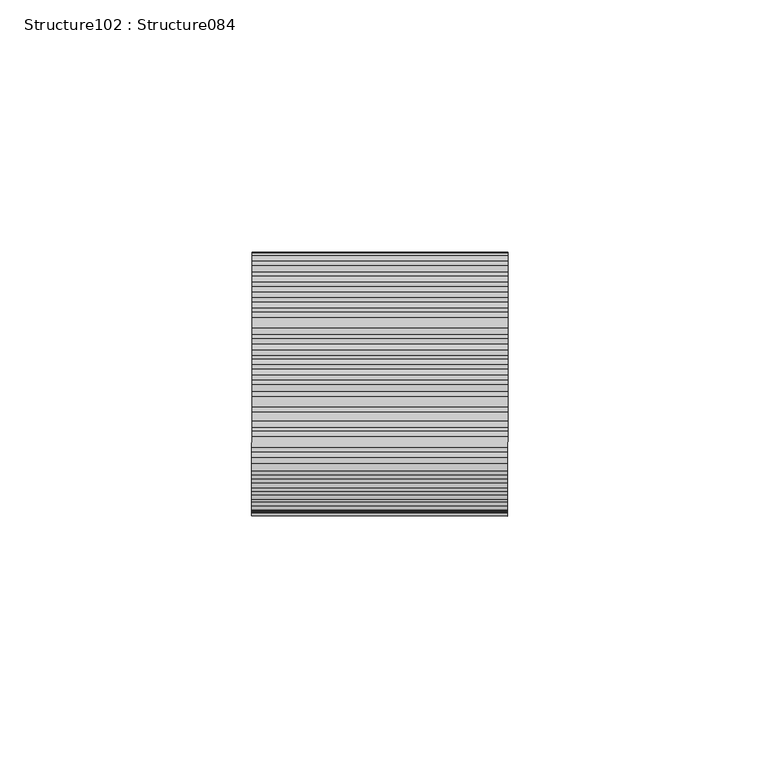
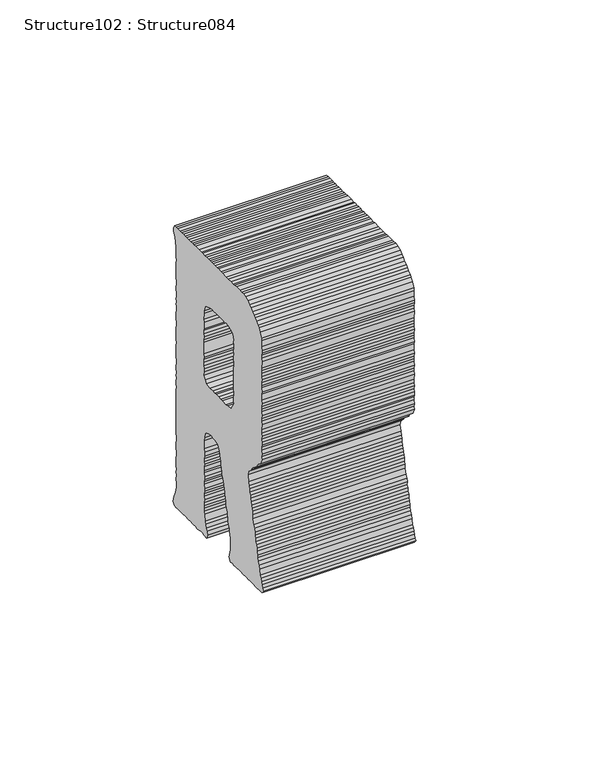
"""IFC4 building model written with IfcOpenShell, lengths in millimetres: proxy geometry, Structure102 : Structure084."""

from ifc_helpers import new_model, si_unit, frame, origin, place, context, project, spatial, polyline, outline, extrude, source, transform, mapped, element, save


def structure102_structure084_8d5e6da8(model_context):
    return source(origin(), model_context, "Body", "SweptSolid", [
        extrude(outline(polyline([(0.7877723, 0.0), (1.9464015, -0.1991228), (2.8602744, -0.2258489), (4.1191818, -0.5725383), (5.014805, -0.7264607), (5.8881786, -1.0119464), (7.2131992, -0.9739456), (7.9618749, -1.2329461), (10.1385127, -1.6070246), (11.3090794, -1.6778663), (12.311293, -1.9804401), (13.2111243, -2.1350857), (14.2117928, -2.4424483), (15.4109212, -2.3828116), (16.5195828, -2.8390667), (17.4342995, -2.8608834), (18.6150357, -2.9334729), (20.3591199, -3.4989322), (21.6394332, -3.7189677), (22.5801144, -3.614914), (23.6845679, -4.0704459), (24.6308599, -3.9673565), (25.7800208, -4.1648521), (26.5039924, -4.5549941), (27.5279624, -4.7309743), (28.8526323, -4.6929132), (29.8357525, -5.1275927), (30.776083, -5.0234788), (32.5416935, -6.2493551), (32.9031424, -7.2342724), (33.5574941, -8.0085019), (34.477038, -8.8236139), (35.0861234, -9.8507291), (35.972525, -11.5876373), (36.8685591, -12.5290416), (37.5229108, -13.303271), (37.9287766, -14.029741), (39.5076035, -14.8278253), (41.6445255, -14.6683322), (42.9644943, -14.6345176), (43.9051754, -14.5304639), (45.0599472, -14.7289238), (46.0220341, -14.4982164), (46.9627152, -14.3941627), (48.1392433, -14.466029), (49.0957798, -14.2340066), (50.041228, -14.1358267), (51.0844997, -14.1847915), (52.1563332, -14.1032778), (53.4327891, -14.3226503), (55.3194114, -14.115447), (56.4288566, -13.7793711), (57.6236345, -13.7240411), (58.7537019, -14.0536423), (59.5858309, -13.7955457), (60.7623592, -13.867412), (61.6189076, -13.4882341), (62.7924221, -13.554528), (63.7358265, -13.4556358), (64.9285003, -13.3999443), (65.8244741, -13.5539269), (66.898061, -13.4727146), (68.1350915, -13.1589264), (69.328609, -13.0983255), (71.318233, -13.0438502), (72.1765349, -12.6649735), (73.2419139, -12.587405), (74.0793029, -12.3302124), (75.2758945, -12.2748331), (76.003044, -11.8734166), (76.8931166, -12.8137963), (76.8480367, -13.8638733), (76.5842472, -14.611004), (76.5400111, -15.6561716), (76.3416115, -16.8105927), (76.0343092, -17.8109105), (75.7045271, -19.7298023), (75.8093424, -20.6702533), (75.3295446, -21.9117003), (75.2811607, -23.7435663), (74.9337097, -25.0027039), (74.4272845, -27.9494233), (74.4005969, -28.8672741), (73.987756, -29.7191213), (74.0707545, -30.7865166), (72.6138584, -31.5939579), (71.7839977, -31.0552851), (70.7821347, -30.7527716), (69.6713689, -30.2961549), (68.9473974, -29.9060129), (66.901912, -29.5544744), (65.7471403, -29.3560146), (64.7624531, -29.7182251), (63.8447229, -29.690836), (62.6738055, -29.6199339), (61.6840006, -29.9762104), (60.4904228, -30.0371621), (59.445047, -29.9878357), (58.3961644, -29.9379066), (57.3516982, -29.893791), (56.362244, -30.2501278), (55.1913266, -30.1792258), (54.145107, -30.1348089), (53.0523006, -30.3383574), (52.1175809, -30.4434355), (51.2156457, -30.2884283), (50.0229718, -30.3441199), (48.9553464, -30.4263568), (47.8617565, -30.634464), (47.0534221, -30.7562085), (45.832477, -30.9427894), (44.914396, -30.91534), (43.7173718, -30.9753383), (42.7766906, -31.079392), (41.494624, -30.8590551), (40.6854459, -30.985709), (39.5926997, -31.1889067), (38.2679695, -31.2273185), (36.4472301, -31.8368423), (35.5455414, -33.266448), (35.3262291, -34.5425532), (34.9408158, -35.2684206), (34.9738469, -36.5929481), (35.1774557, -38.4731762), (35.8364483, -39.2435097), (37.3094464, -39.8927126), (38.4142507, -40.3483048), (41.3574633, -40.8541273), (42.4292967, -40.7726136), (43.70961, -40.9926491), (44.6888727, -41.4266656), (45.7377553, -41.4765946), (46.525177, -41.4765343), (47.5244428, -41.7836559), (48.8103669, -42.0046557), (49.6810775, -42.2846293), (50.8784525, -42.2246912), (51.9076827, -42.4015754), (52.649904, -42.6645211), (53.6552737, -42.9676373), (54.9802942, -42.9296365), (56.0035629, -43.1054961), (56.8555307, -43.5176357), (57.7515045, -43.6716183), (58.9488796, -43.6116803), (60.0554372, -44.0675738), (61.0990598, -44.1165988), (61.869492, -44.2490058), (63.0007539, -44.5737579), (63.9372269, -44.468981), (66.2885299, -44.6124123), (67.125919, -44.3552198), (68.4493124, -44.3266871), (69.3028472, -43.9419367), (70.5019756, -43.8823001), (71.6935756, -44.6185287), (71.3461245, -45.8776663), (70.9132807, -46.8564085), (70.759298, -47.7523823), (70.7307966, -48.6702824), (70.6639602, -49.846953), (70.3566579, -50.8472708), (70.3341179, -51.7661956), (70.157535, -52.7936724), (69.7472914, -53.6409116), (69.69625, -54.689964), (69.3228948, -56.8623937), (69.2778149, -57.9124707), (68.992269, -58.786195), (68.6181303, -60.9631834), (68.5955903, -61.882108), (68.4416077, -62.7780818), (67.1345464, -63.4762478), (66.0458878, -62.8930979), (65.1969939, -62.4861801), (64.1318451, -61.7767379), (63.4057694, -61.3862343), (61.4454907, -60.5179), (60.4218712, -60.34198), (58.3267691, -60.2476341), (57.4807627, -59.8365191), (56.1757452, -59.747625), (55.2985141, -59.4614764), (54.2305381, -59.5436531), (51.2834681, -59.0371676), (50.3063094, -58.6035127), (49.28269, -58.4275928), (47.9738151, -58.3380358), (46.0598327, -58.0090974), (45.0553067, -57.7010718), (44.0334407, -57.5254533), (42.9872211, -57.4810363), (39.0186357, -56.7989926), (37.9732599, -56.7496662), (36.9678902, -56.4465501), (35.6637165, -56.3527465), (34.6422011, -56.1771882), (33.8931746, -55.9181273), (32.8499028, -55.8691626), (31.563628, -55.6481025), (30.5617652, -55.345589), (29.6714021, -55.1925706), (28.7480611, -55.1642173), (27.5989002, -54.9667217), (26.7434256, -54.5539795), (25.5695604, -54.4876253), (24.5262885, -54.4386606), (23.4214843, -53.9830685), (22.6245944, -53.9815015), (21.6235752, -53.6740786), (20.3206618, -53.5855461), (19.2756365, -53.53628), (18.5509637, -53.1460175), (17.268897, -52.9256806), (16.4593683, -53.0522742), (15.300739, -52.8531514), (14.4321325, -52.5735394), (13.3871074, -52.5242734), (12.1225891, -52.1766197), (11.3803678, -51.913674), (10.2086067, -51.8476814), (8.0263581, -51.4726387), (7.2362735, -51.4671869), (6.1085182, -51.1430374), (5.2354954, -50.8576121), (4.0800223, -50.6590317), (3.1400425, -50.7632058), (2.0122874, -50.4390564), (1.0892969, -50.4107633), (-0.1431529, -49.9332339), (-1.1706297, -49.7566511), (-2.2147453, -49.7125957), (-2.9573172, -49.4495897), (-4.0087969, -49.4042688), (-5.0080628, -49.0971472), (-6.2887267, -48.8770514), (-7.1035156, -49.002741), (-8.3620724, -48.6561119), (-9.1102552, -48.3921416), (-10.1314198, -48.2166436), (-11.1997466, -48.29876), (-12.2051163, -47.9956438), (-13.4854295, -47.7756083), (-14.2776182, -47.7697949), (-16.3227529, -47.4183166), (-17.4331681, -46.9617602), (-18.4993908, -47.0442382), (-19.6267952, -46.720149), (-20.6781325, -46.6697981), (-21.5523499, -46.3892219), (-23.7729936, -46.2733003), (-24.8401259, -46.3505675), (-25.6975181, -46.7346549), (-26.7864672, -46.9388664), (-27.9612419, -46.8673015), (-28.903386, -46.1836923), (-28.8523447, -45.1346398), (-28.6983018, -44.2383154), (-28.3526042, -42.9788764), (-28.220378, -42.2094962), (-28.1483637, -41.0384089), (-27.8679957, -40.1591013), (-27.8177379, -39.1146076), (-27.6201821, -37.965096), (-27.3406578, -37.0906979), (-27.2677998, -35.9147012), (-27.010032, -35.1668965), (-26.9597742, -34.1224028), (-26.6073919, -32.0720079), (-26.2616943, -30.812569), (-26.3826552, -29.9996758), (-25.9319123, -28.8936771), (-25.9875435, -27.7006526), (-25.6832549, -26.6947624), (-25.4254871, -25.9469578), (-25.5028748, -24.8805269), (-25.2212466, -24.0064903), (-25.1513363, -22.8350415), (-24.8470476, -21.8291512), (-24.8207105, -20.9112402), (-24.3473674, -19.6737385), (-24.2963261, -18.624686), (-23.8191857, -16.6004256), (-23.6434466, -15.5778582), (-23.3571774, -13.9121534), (-23.1370214, -12.6311388), (-23.1311202, -11.8447417), (-23.0821829, -10.7953276), (-22.707984, -8.6179885), (-22.4263557, -7.743952), (-22.3782019, -6.6990967), (-21.9266152, -5.5881886), (-21.1449177, -4.1383221), (-20.1224106, -3.5266396), (-19.3473977, -2.8677291), (-18.3143703, -2.2578546), (-17.5002006, -1.3395928), (-16.8785895, -0.7897057), (-16.003649, -0.2783015), (-15.0749656, 0.4848928), (-14.3537777, 0.887334), (-13.1940143, 1.480482), (-11.3979792, 1.9588644), (-10.4794051, 1.9363848), (-8.428309, 1.583882), (-7.1300967, 1.491103), (-6.3554563, 1.3579728), (-5.3765442, 0.9240165), (-4.3546782, 0.7483979), (-3.2867022, 0.8305746), (-1.0232687, 0.1758597), (0.0, 0.0), (0.7877723, 0.0)]), holes=[polyline([(18.9318371, -31.7250019), (19.2826525, -30.4714969), (19.2842194, -29.6746071), (19.5035317, -28.3985019), (19.9610799, -27.2886183), (20.0100172, -26.2392042), (20.4892615, -24.2153054), (20.3840956, -23.2747941), (20.4678464, -21.3085647), (19.6312408, -20.7734262), (18.3769139, -19.6354193), (17.4595343, -19.6080904), (16.1792211, -19.3880549), (15.4301946, -19.1289941), (14.2771763, -18.9308356), (13.3629527, -18.9040491), (12.3417881, -18.7285511), (11.0337569, -18.6340846), (8.9865181, -18.2822447), (7.9811484, -17.9791286), (7.0630675, -17.9516792), (6.1670937, -17.7976965), (5.0614456, -17.3470139), (4.1654718, -17.1930312), (2.9889437, -17.1211649), (2.0926191, -16.9671219), (1.0925096, -16.6649099), (-0.0840186, -16.5930435), (-0.958236, -16.3124674), (-2.1130076, -16.1140075), (-3.0310886, -16.086558), (-3.8996952, -15.8069462), (-5.549276, -16.1852201), (-6.4511511, -16.8176346), (-7.5496121, -18.6044207), (-7.7253512, -19.6269881), (-7.6009438, -20.4408347), (-8.0334371, -21.4196371), (-8.5841586, -24.6241024), (-8.6784224, -25.9267529), (-8.6799072, -26.7189635), (-9.1123403, -27.6974153), (-9.0314457, -28.7644489), (-8.7006845, -30.6715839), (-8.3169861, -31.524938), (-6.8689006, -32.3001919), (-5.9732775, -32.4541143), (-3.7094934, -33.1088895), (-2.7730203, -33.0041127), (-0.5967332, -33.3781309), (0.1279397, -33.7683934), (1.3044679, -33.8402597), (2.2230419, -33.8627393), (3.4554917, -34.3402687), (4.2455764, -34.3457206), (8.2162658, -35.0281259), (9.3915337, -35.0947212), (10.2435015, -35.5068607), (11.272381, -35.6836846), (12.4436491, -35.7546469), (13.3625738, -35.7771868), (14.3896999, -35.9537094), (15.6435555, -36.304585), (17.0346893, -35.8818941), (18.0463108, -35.3986733), (18.8829602, -33.5618376), (18.9318371, -31.7250019)])]), frame((-56111.8259032, 290611.5615484, -297.3854876), z_axis=(-0.9999998917542984, 0.00046528635450596156, 0.0), x_axis=(-7.880904225957716e-05, -0.16937748758385043, -0.9855512470130193)), (0.0, 0.0, 1.0), 50.8),
    ])


if __name__ == "__main__":
    model = new_model("IFC4")
    model_context = context("Model", 3, world=origin())
    ifc_project = project(units=[si_unit("LENGTHUNIT", "METRE", prefix="MILLI")], contexts=[model_context])
    site = spatial("IfcSite", under=ifc_project)
    building = spatial("IfcBuilding", under=site)
    placement = place(None, origin())
    structure102_structure084_shape = structure102_structure084_8d5e6da8(model_context)
    element("IfcBuildingElementProxy", 1, Name="Structure102 : Structure084", ObjectType="Structure102 : Structure084", at=placement, inside=building, context=model_context, shape_type="MappedRepresentation", body=[
        mapped(structure102_structure084_shape, transform((0.0, 0.0, 0.0), x_axis=(1.0, 0.0, 0.0), y_axis=(0.0, 1.0, 0.0), z_axis=(0.0, 0.0, 1.0))),
    ])
    save(model, "model.ifc")

# Revit data of these elements
# Type "Structure102 : Structure084"
#   NameOverride = "Structure084"
# Element 1 (IfcBuildingElementProxy, "Structure102 : Structure084")
#   Materials on its faces: "BRUSHED ALUMINUM LETTERING"
# Materials
#   "BRUSHED ALUMINUM LETTERING": class "Unassigned", colour RGB 169 181 186, transparency 0, Cost = 0
